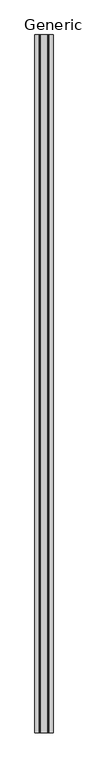
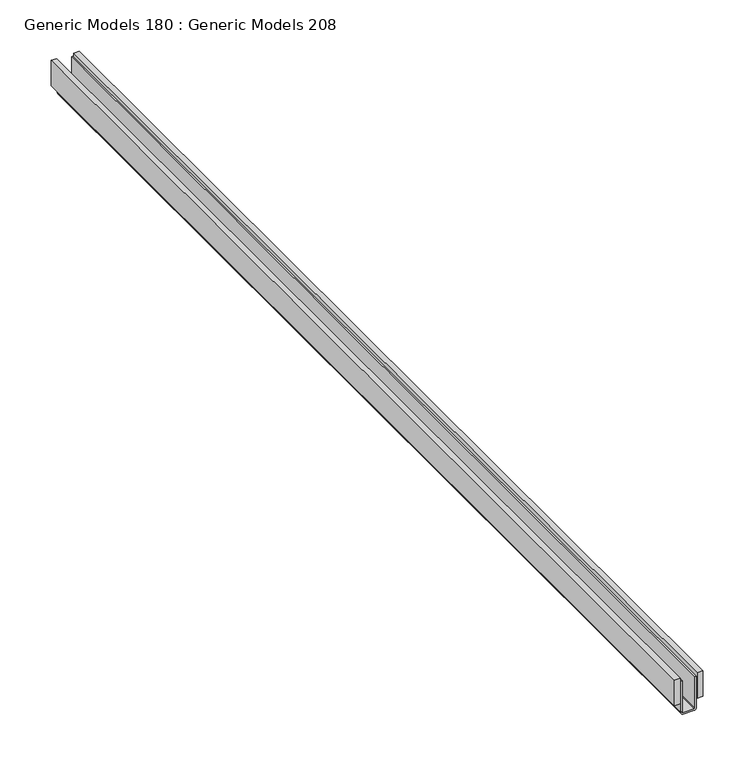
"""IFC4 building model written with IfcOpenShell, lengths in millimetres: proxy geometry, Generic Models 180 : Generic Models 208."""

from ifc_helpers import new_model, si_unit, point, frame, frame_2d, origin, place, context, project, spatial, polyline, circle_curve, trimmed, segment, composite_curve, outline, extrude, source, transform, mapped, element, save


def generic_models_180_generic_models_208_d2dc2d15(model_context):
    return source(origin(), model_context, "Body", "SweptSolid", [
        extrude(outline(polyline([(53745.8524408, -228.7033818), (53739.5024408, -228.7033818), (53739.5024408, 990.4966182), (53745.8524408, 990.4966182), (53745.8524408, -228.7033818)])), frame((0.0, 0.0, 2074.6253412), z_axis=(0.0, 0.0, 1.0), x_axis=(1.0, 0.0, 0.0)), (0.0, 0.0, 1.0), 30.1625),
        extrude(outline(composite_curve([segment(polyline([(2063.4947557, 53738.7086908), (2101.0175287, 53738.7086908), (2101.0175287, 53737.1211908), (2063.4947557, 53737.1211908)]), True, "CONTINUOUS"), segment(trimmed(circle_curve(frame_2d((2063.4947557, 53736.3455263)), 0.7756645), [point((2063.4947557, 53737.1211908))], [point((2062.7190912, 53736.3455263))], True, "CARTESIAN"), True, "CONTINUOUS"), segment(polyline([(2062.7190912, 53736.3455263), (2062.7190912, 53723.6258979)]), True, "CONTINUOUS"), segment(trimmed(circle_curve(frame_2d((2063.5112983, 53723.6258979)), 0.792207), [point((2062.7190912, 53723.6258979))], [point((2063.5112983, 53722.8336908))], True, "CARTESIAN"), True, "CONTINUOUS"), segment(polyline([(2063.5112983, 53722.8336908), (2101.0175287, 53722.8336908), (2101.0175287, 53721.2461908), (2063.5112983, 53721.2461908)]), True, "CONTINUOUS"), segment(trimmed(circle_curve(frame_2d((2063.5112983, 53723.6258979)), 2.379707), [point((2063.5112983, 53721.2461908))], [point((2061.1315912, 53723.6258979))], False, "CARTESIAN"), True, "CONTINUOUS"), segment(polyline([(2061.1315912, 53723.6258979), (2061.1315912, 53736.3455263)]), True, "CONTINUOUS"), segment(trimmed(circle_curve(frame_2d((2063.4947557, 53736.3455263)), 2.3631645), [point((2061.1315912, 53736.3455263))], [point((2063.4947557, 53738.7086908))], False, "CARTESIAN"), True, "CONTINUOUS")], self_intersect=False)), frame((0.0, -228.7033818, 0.0), z_axis=(0.0, 1.0, 0.0), x_axis=(0.0, 0.0, 1.0)), (0.0, 0.0, 1.0), 1219.2),
        extrude(outline(polyline([(53720.4524408, -228.7033818), (53714.1024408, -228.7033818), (53714.1024408, 990.4966182), (53720.4524408, 990.4966182), (53720.4524408, -228.7033818)])), frame((0.0, 0.0, 2074.6253412), z_axis=(0.0, 0.0, 1.0), x_axis=(1.0, 0.0, 0.0)), (0.0, 0.0, 1.0), 30.1625),
    ])


if __name__ == "__main__":
    model = new_model("IFC4")
    model_context = context("Model", 3, world=origin())
    ifc_project = project(units=[si_unit("LENGTHUNIT", "METRE", prefix="MILLI")], contexts=[model_context])
    site = spatial("IfcSite", under=ifc_project)
    building = spatial("IfcBuilding", under=site)
    placement = place(None, origin())
    generic_models_180_generic_models_208_shape = generic_models_180_generic_models_208_d2dc2d15(model_context)
    element("IfcBuildingElementProxy", 1, Name="Generic Models 180 : Generic Models 208", ObjectType="Generic Models 180 : Generic Models 208", at=placement, inside=building, context=model_context, shape_type="MappedRepresentation", body=[
        mapped(generic_models_180_generic_models_208_shape, transform((0.0, 0.0, 0.0), x_axis=(1.0, 0.0, 0.0), y_axis=(0.0, 1.0, 0.0), z_axis=(0.0, 0.0, 1.0))),
    ])
    save(model, "model.ifc")

# Revit data of these elements
# Element 1 (IfcBuildingElementProxy, "Generic Models 180 : Generic Models 208")
#   Materials on its faces: "UNISTRUT P2750  -1-5/8\" X 1/4\", 4 WHEEL TROLLEY"
# Materials
#   "UNISTRUT P2750  -1-5/8\" X 1/4\", 4 WHEEL TROLLEY": class "Metal", colour RGB 244 244 244, transparency 0, Description = "Aluminum 6061", Cost = 0
